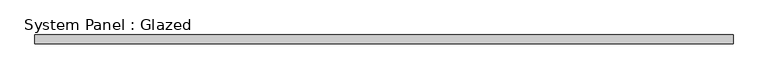
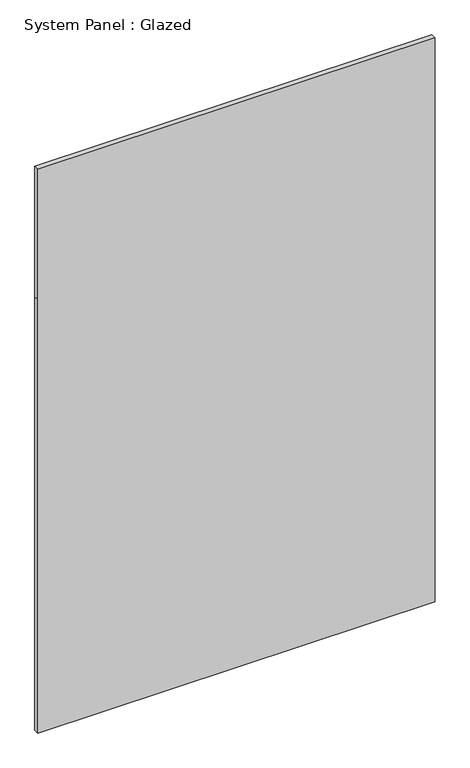
"""IFC4 building model written with IfcOpenShell, lengths in millimetres: plate geometry, System Panel : Glazed."""

from ifc_helpers import new_model, si_unit, frame, origin, place, context, project, spatial, polyline, outline, extrude, source, transform, mapped, element, save


def system_panel_glazed_3bc425d8(model_context):
    return source(origin(), model_context, "Body", "SweptSolid", [
        extrude(outline(polyline([(0.0, -975.0), (0.0, 975.0), (2250.0, 975.0), (2925.0, 975.0), (2925.0, -975.0), (2250.0, -975.0), (0.0, -975.0)])), frame((0.0, 24.5, 0.0), z_axis=(0.0, 1.0, 0.0), x_axis=(0.0, 0.0, 1.0)), (0.0, 0.0, 1.0), 25.0),
    ])


if __name__ == "__main__":
    model = new_model("IFC4")
    model_context = context("Model", 3, world=origin())
    ifc_project = project(units=[si_unit("LENGTHUNIT", "METRE", prefix="MILLI")], contexts=[model_context])
    site = spatial("IfcSite", under=ifc_project)
    building = spatial("IfcBuilding", under=site)
    placement = place(None, origin())
    system_panel_glazed_shape = system_panel_glazed_3bc425d8(model_context)
    element("IfcPlate", 1, ObjectType="System Panel : Glazed", at=placement, inside=building, context=model_context, shape_type="MappedRepresentation", body=[
        mapped(system_panel_glazed_shape, transform((0.0, 0.0, 0.0), x_axis=(1.0, 0.0, 0.0), y_axis=(0.0, 1.0, 0.0), z_axis=(0.0, 0.0, 1.0))),
    ])
    save(model, "model.ifc")

# Revit data of these elements
# Element 1 (IfcPlate, "System Panel : Glazed")
#   Materials on its faces: "Glass"
# Materials
#   "Glass": class "Glass", colour RGB 0 128 192, transparency 0.9
